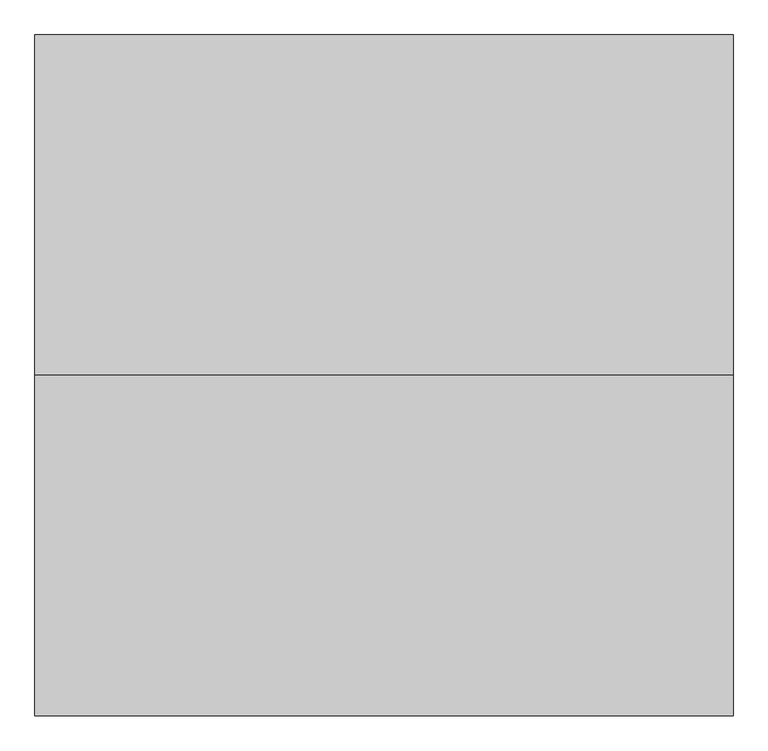
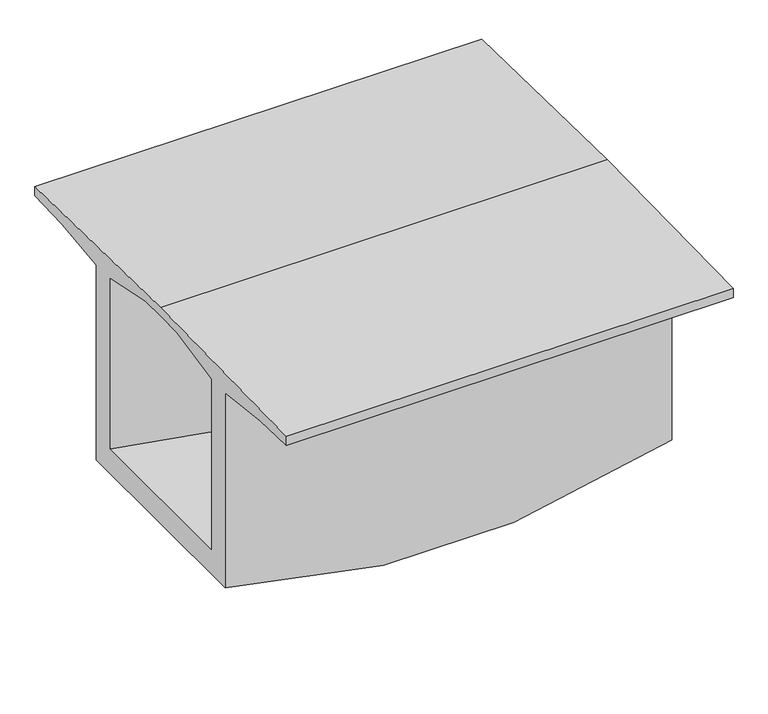
"""IFC4 building model written with IfcOpenShell, lengths in millimetres: proxy geometry, K1+K0+K1_2 : K1+K0+K1_2."""

from ifc_helpers import new_model, si_unit, frame, origin, place, context, project, spatial, source, transform, mapped, element, save
from ifc_brep_helpers import plane_surface, spline_surface, advanced_brep


def generic_models_2616fa81(model_context):
    return source(origin(), model_context, "Body", "AdvancedBrep", [
        advanced_brep(
        [(-6000.0, 5850.0, -367.0), (-6000.0, 5850.0, -117.0), (6000.0, 5850.0, -117.0), (6000.0, 5850.0, -367.0), (-6000.0, 4600.0, -421.0), (6000.0, 4599.9997971, -420.9953034), (-6000.0, 3000.0, -607.0), (6000.0, 2999.9994603, -606.9953573), (-1750.0, 3000.0, -6999.9983335), (-6000.0, 3000.0, -6150.0), (6000.0, 3000.0, -6150.0), (1750.0, 3000.0, -6999.9983335), (-1750.0, -3000.0, -6999.9983335), (-6000.0, -3000.0, -6150.0), (1750.0, -3000.0, -6999.9983335), (6000.0, -3000.0, -6150.0), (6000.0, -3000.0, -607.0), (-6000.0, -3000.0, -607.0), (-6000.0, -4600.0, -421.0), (6000.0, -4599.9994603, -420.9953573), (-6000.0, -5850.0, -367.0), (6000.0, -5849.9997971, -366.9953034), (-6000.0, -5850.0, -117.0), (6000.0, -5850.0, -117.0), (-6000.0, 0.0, 0.0), (6000.0, -9.41e-05, 0.0047035), (-6000.0, -2350.0, -5450.0), (-6000.0, 2350.0, -5450.0), (-6000.0, 2350.0, -607.0), (-6000.0, 750.0, -265.0), (-6000.0, 0.0, -250.0), (-6000.0, -750.0, -265.0), (-6000.0, -2350.0, -607.0), (-1750.0, -2100.0, -5999.9983335), (-2750.0, -2350.0, -5999.9983335), (-2750.0, -2350.0, -606.9983335), (-1750.0, -2100.0, -856.9983335), (-2750.0, -750.0, -264.9983335), (-1750.0, -750.0, -514.9983335), (-2750.0, 0.0, -249.9983335), (-1750.0, 0.0, -499.9983335), (-2750.0, 750.0, -264.9983335), (-1750.0, 750.0, -514.9983335), (-2750.0, 2350.0, -606.9983335), (-1750.0, 2100.0, -856.9983335), (-2750.0, 2350.0, -5999.9983335), (-1750.0, 2100.0, -5999.9983335), (-1750.0, 400.0, -5999.9983335), (-1750.0, 500.0, -5899.9983335), (-1750.0, 500.0, -4099.9983335), (-1750.0, 400.0, -3999.9983335), (-1750.0, -400.0, -3999.9983335), (-1750.0, -500.0, -4099.9983335), (-1750.0, -500.0, -5899.9983335), (-1750.0, -400.0, -5999.9983335), (1750.0, -400.0, -5999.9983335), (1750.0, -500.0, -5899.9983335), (1750.0, -500.0, -4099.9983335), (1750.0, -400.0, -3999.9983335), (1750.0, 400.0, -3999.9983335), (1750.0, 500.0, -4099.9983335), (1750.0, 500.0, -5899.9983335), (1750.0, 400.0, -5999.9983335), (1750.0, 2100.0, -5999.9983335), (1750.0, 2100.0, -856.9983335), (1750.0, 750.0, -514.9983335), (1750.0, 0.0, -499.9983335), (1750.0, -750.0, -514.9983335), (1750.0, -2100.0, -856.9983335), (1750.0, -2100.0, -5999.9983335), (2750.0, -2350.0, -5999.9983335), (2750.0, 2350.0, -5999.9983335), (6000.0, 2350.0, -607.0), (6000.0, 2350.0, -5450.0), (6000.0, -2350.0, -5450.0), (6000.0, -2350.0, -607.0), (6000.0, -750.0, -265.0), (6000.0, 0.0, -250.0), (6000.0, 750.0, -265.0), (2750.0, 2350.0, -606.9983335), (2750.0, 750.0, -264.9983335), (2750.0, 0.0, -249.9983335), (2750.0, -750.0, -264.9983335), (2750.0, -2350.0, -606.9983335)],
        [
            (0, 1),
            (1, 2),
            (2, 3),
            (3, 0),
            (4, 0),
            (3, 5),
            (5, 4),
            (6, 4),
            (5, 7),
            (7, 6),
            (8, 9),
            (9, 6),
            (7, 10),
            (10, 11),
            (11, 8),
            (8, 12),
            (12, 13),
            (13, 9),
            (12, 14),
            (14, 15),
            (15, 16),
            (16, 17),
            (17, 13),
            (18, 17),
            (16, 19),
            (19, 18),
            (20, 18),
            (19, 21),
            (21, 20),
            (22, 20),
            (21, 23),
            (23, 22),
            (24, 22),
            (23, 25),
            (25, 24),
            (1, 24),
            (25, 2),
            (26, 27),
            (27, 28),
            (28, 29),
            (29, 30),
            (30, 31),
            (31, 32),
            (32, 26),
            (33, 34),
            (34, 35),
            (35, 36),
            (36, 33),
            (35, 37),
            (37, 38),
            (38, 36),
            (37, 39),
            (39, 40),
            (40, 38),
            (39, 41),
            (41, 42),
            (42, 40),
            (41, 43),
            (43, 44),
            (44, 42),
            (45, 46),
            (46, 44),
            (43, 45),
            (46, 47),
            (47, 48),
            (48, 49),
            (49, 50),
            (50, 51),
            (51, 52),
            (52, 53),
            (53, 54),
            (54, 33),
            (45, 27),
            (26, 34),
            (34, 45),
            (32, 35),
            (31, 37),
            (30, 39),
            (29, 41),
            (28, 43),
            (11, 14),
            (55, 56),
            (56, 57),
            (57, 58),
            (58, 59),
            (59, 60),
            (60, 61),
            (61, 62),
            (62, 63),
            (63, 64),
            (64, 65),
            (65, 66),
            (66, 67),
            (67, 68),
            (68, 69),
            (69, 55),
            (53, 56),
            (55, 54),
            (69, 70),
            (70, 71),
            (71, 63),
            (62, 47),
            (61, 48),
            (60, 49),
            (59, 50),
            (58, 51),
            (57, 52),
            (10, 15),
            (72, 73),
            (73, 74),
            (74, 75),
            (75, 76),
            (76, 77),
            (77, 78),
            (78, 72),
            (71, 73),
            (72, 79),
            (79, 71),
            (78, 80),
            (80, 79),
            (77, 81),
            (81, 80),
            (76, 82),
            (82, 81),
            (75, 83),
            (83, 82),
            (74, 70),
            (70, 83),
            (79, 64),
            (80, 65),
            (81, 66),
            (82, 67),
            (83, 68),
        ],
        [
            plane_surface(frame((-1750.0, 5850.0, -241.9983335), z_axis=(0.0, 1.0, 0.0), x_axis=(0.0, 0.0, -1.0))),
            plane_surface(frame((-1750.0, 5225.0, -393.9983335), z_axis=(3.917521675919369e-07, 0.043159745550590725, -0.9990681840414372), x_axis=(0.0, -0.9990681840415138, -0.043159745550594035))),
            plane_surface(frame((-1750.0, 3800.0, -513.9983335), z_axis=(3.8949455357734467e-07, 0.11547236802580216, -0.9933106926950712), x_axis=(0.0, -0.9933106926951465, -0.11547236802581091))),
            plane_surface(frame((-1750.0, 3000.0, -3803.4983335), z_axis=(0.0, 1.0, 0.0), x_axis=(0.0, 0.0, -1.0))),
            plane_surface(frame((-1750.0, 0.0, -6999.9983335), z_axis=(-0.1961157654238259, 0.0, -0.9805807496337193), x_axis=(0.0, -1.0, 0.0))),
            plane_surface(frame((-1750.0, -3000.0, -3803.4983335), z_axis=(0.0, -1.0, 0.0), x_axis=(0.0, 0.0, 1.0))),
            plane_surface(frame((-1750.0, -3800.0, -513.9983335), z_axis=(3.8949455045787845e-07, -0.11547236802580199, -0.9933106926950712), x_axis=(0.0, -0.9933106926951465, 0.11547236802581075))),
            plane_surface(frame((-1750.0, -5225.0, -393.9983335), z_axis=(3.917521632228593e-07, -0.043159745550590524, -0.9990681840414372), x_axis=(0.0, -0.9990681840415138, 0.043159745550593834))),
            plane_surface(frame((-1750.0, -5850.0, -241.9983335), z_axis=(0.0, -1.0, 0.0), x_axis=(0.0, 0.0, 1.0))),
            plane_surface(frame((-1750.0, -2925.0, -58.4983335), z_axis=(-3.920391455849865e-07, -0.019996001199585858, 0.9998000599799306), x_axis=(0.0, 0.9998000599800073, 0.01999600119958739))),
            plane_surface(frame((-1750.0, 2925.0, -58.4983335), z_axis=(-3.9203914802891097e-07, 0.0199960011995859, 0.9998000599799306), x_axis=(0.0, 0.9998000599800073, -0.019996001199587433))),
            plane_surface(frame((-6000.0, 0.0, -1393.0909091), z_axis=(-1.0, 0.0, 0.0), x_axis=(0.0, 0.0, -1.0))),
            plane_surface(frame((-1750.0, -2100.0, -3428.4983335), z_axis=(-0.24253562503633255, 0.970142500145332, 0.0), x_axis=(0.0, 0.0, 1.0))),
            spline_surface(1, 1, [[(-1750.0, -2100.0, -856.9983335), (-1750.0, -750.0, -514.9983335)], [(-2750.0, -2350.0, -606.9983335), (-2750.0, -750.0, -264.9983335)]], [2, 2], [2, 2], [0.0, 1.0], [0.0, 1.0]),
            plane_surface(frame((-1750.0, -375.0, -507.4983335), z_axis=(-0.24248998415805265, 0.019399198732549593, -0.9699599366322108), x_axis=(0.0, 0.999800059980009, 0.019996001199502643))),
            plane_surface(frame((-1750.0, 375.0, -507.4983335), z_axis=(-0.2424899841580526, -0.019399198732545083, -0.969959936632211), x_axis=(0.0, 0.9998000599800091, -0.019996001199497994))),
            spline_surface(1, 1, [[(-1750.0, 750.0, -514.9983335), (-1750.0, 2100.0, -856.9983335)], [(-2750.0, 750.0, -264.9983335), (-2750.0, 2350.0, -606.9983335)]], [2, 2], [2, 2], [0.0, 1.0], [0.0, 1.0]),
            plane_surface(frame((-1750.0, 2100.0, -3428.4983335), z_axis=(-0.2425356250363329, -0.970142500145332, 0.0), x_axis=(0.0, 0.0, -1.0))),
            plane_surface(frame((-1750.0, 0.0, -2177.7126192), z_axis=(-1.0, 0.0, 0.0), x_axis=(0.0, 0.0, 1.0))),
            plane_surface(frame((-2750.0, 0.0, -5999.9983335), z_axis=(0.16685781218853318, 0.0, 0.9859809686356306), x_axis=(0.0, -1.0, 0.0))),
            plane_surface(frame((-2750.0, -2350.0, -3303.4983335), z_axis=(0.0, 1.0, 0.0), x_axis=(0.0, 0.0, 1.0))),
            plane_surface(frame((-2750.0, -1550.0, -435.9983335), z_axis=(5.014418331334979e-07, 0.2090281807047397, -0.9779096173323053), x_axis=(0.0, 0.9779096173324281, 0.20902818070476595))),
            plane_surface(frame((-2750.0, -375.0, -257.4983335), z_axis=(5.126665763907822e-07, 0.01999600119949824, -0.9998000599798776), x_axis=(0.0, 0.999800059980009, 0.019996001199500867))),
            plane_surface(frame((-2750.0, 375.0, -257.4983335), z_axis=(5.126665768021895e-07, -0.01999600119949714, -0.9998000599798776), x_axis=(0.0, 0.999800059980009, -0.019996001199499767))),
            plane_surface(frame((-2750.0, 1550.0, -435.9983335), z_axis=(5.014418348904322e-07, -0.209028180704739, -0.9779096173323053), x_axis=(0.0, 0.9779096173324282, -0.20902818070476525))),
            plane_surface(frame((-2750.0, 2350.0, -3303.4983335), z_axis=(0.0, -1.0, 0.0), x_axis=(0.0, 0.0, -1.0))),
            plane_surface(frame((-1750.0, 0.0, -6999.9983335), z_axis=(0.0, 0.0, -1.0), x_axis=(0.0, 1.0, 0.0))),
            plane_surface(frame((1750.0, 0.0, -1547.6346971), z_axis=(1.0, 0.0, 0.0), x_axis=(0.0, -0.9998000599800073, 0.019996001199585656))),
            plane_surface(frame((-1750.0, -450.0, -5949.9983335), z_axis=(0.0, 0.7071067811866191, 0.7071067811864761), x_axis=(0.0, 0.7071067811864761, -0.7071067811866191))),
            plane_surface(frame((-1750.0, 0.0, -5999.9983335), z_axis=(0.0, 0.0, 1.0), x_axis=(0.0, 1.0, 0.0))),
            plane_surface(frame((-1750.0, 450.0, -5949.9983335), z_axis=(0.0, -0.7071067811866215, 0.7071067811864736), x_axis=(0.0, 0.7071067811864736, 0.7071067811866215))),
            plane_surface(frame((-1750.0, 500.0, -4999.9983335), z_axis=(0.0, -1.0, 0.0), x_axis=(0.0, 0.0, 1.0))),
            plane_surface(frame((-1750.0, 450.0, -4049.9983335), z_axis=(0.0, -0.707106781186443, -0.7071067811866522), x_axis=(0.0, -0.7071067811866522, 0.707106781186443))),
            plane_surface(frame((-1750.0, 0.0, -3999.9983335), z_axis=(0.0, 0.0, -1.0), x_axis=(0.0, -1.0, 0.0))),
            plane_surface(frame((-1750.0, -450.0, -4049.9983335), z_axis=(0.0, 0.7071067811864454, -0.7071067811866497), x_axis=(0.0, -0.7071067811866497, -0.7071067811864454))),
            plane_surface(frame((-1750.0, -500.0, -4999.9983335), z_axis=(0.0, 1.0, 0.0), x_axis=(0.0, 0.0, -1.0))),
            plane_surface(frame((1750.0, 0.0, -6999.9983335), z_axis=(0.1961157654238259, 0.0, -0.9805807496337193), x_axis=(0.0, 1.0, 0.0))),
            plane_surface(frame((6000.0, 0.0, -1393.0909091), z_axis=(1.0000000000000002, 0.0, 0.0), x_axis=(0.0, -0.9998000599800073, 0.019996001199587433))),
            plane_surface(frame((2750.0, 2350.0, -3303.4983335), z_axis=(0.0, -1.0, 0.0), x_axis=(0.0, 0.0, 1.0))),
            plane_surface(frame((2750.0, 1550.0, -435.9983335), z_axis=(-5.014418348904322e-07, -0.209028180704739, -0.9779096173323053), x_axis=(0.0, -0.9779096173324282, 0.20902818070476525))),
            plane_surface(frame((2750.0, 375.0, -257.4983335), z_axis=(-5.126665768021895e-07, -0.01999600119949714, -0.9998000599798776), x_axis=(0.0, -0.999800059980009, 0.019996001199499767))),
            plane_surface(frame((2750.0, -375.0, -257.4983335), z_axis=(-5.126665763907822e-07, 0.01999600119949824, -0.9998000599798776), x_axis=(0.0, -0.999800059980009, -0.019996001199500867))),
            plane_surface(frame((2750.0, -1550.0, -435.9983335), z_axis=(-5.014418331334979e-07, 0.2090281807047397, -0.9779096173323053), x_axis=(0.0, -0.9779096173324281, -0.20902818070476595))),
            plane_surface(frame((2750.0, -2350.0, -3303.4983335), z_axis=(0.0, 1.0, 0.0), x_axis=(0.0, 0.0, -1.0))),
            plane_surface(frame((2750.0, 0.0, -5999.9983335), z_axis=(-0.16685781218853318, 0.0, 0.9859809686356306), x_axis=(0.0, 1.0, 0.0))),
            plane_surface(frame((1750.0, 2100.0, -3428.4983335), z_axis=(0.2425356250363329, -0.970142500145332, 0.0), x_axis=(0.0, 0.0, 1.0))),
            spline_surface(1, 1, [[(1750.0, 2100.0, -856.9983335), (1750.0, 750.0, -514.9983335)], [(2750.0, 2350.0, -606.9983335), (2750.0, 750.0, -264.9983335)]], [2, 2], [2, 2], [0.0, 1.0], [0.0, 1.0]),
            plane_surface(frame((1750.0, 375.0, -507.4983335), z_axis=(0.2424899841580526, -0.019399198732545083, -0.969959936632211), x_axis=(0.0, -0.9998000599800091, 0.019996001199497994))),
            plane_surface(frame((1750.0, -375.0, -507.4983335), z_axis=(0.24248998415805265, 0.019399198732549593, -0.9699599366322108), x_axis=(0.0, -0.999800059980009, -0.019996001199502643))),
            spline_surface(1, 1, [[(1750.0, -750.0, -514.9983335), (1750.0, -2100.0, -856.9983335)], [(2750.0, -750.0, -264.9983335), (2750.0, -2350.0, -606.9983335)]], [2, 2], [2, 2], [0.0, 1.0], [0.0, 1.0]),
            plane_surface(frame((1750.0, -2100.0, -3428.4983335), z_axis=(0.24253562503633255, 0.970142500145332, 0.0), x_axis=(0.0, 0.0, -1.0))),
        ],
        [
            (0, [[1, 2, 3, 4]]),
            (1, [[5, -4, 6, 7]]),
            (2, [[8, -7, 9, 10]]),
            (3, [[11, 12, -10, 13, 14, 15]]),
            (4, [[-11, 16, 17, 18]]),
            (5, [[-17, 19, 20, 21, 22, 23]]),
            (6, [[24, -22, 25, 26]]),
            (7, [[27, -26, 28, 29]]),
            (8, [[30, -29, 31, 32]]),
            (9, [[33, -32, 34, 35]]),
            (10, [[-2, 36, -35, 37]]),
            (11, [[-1, -5, -8, -12, -18, -23, -24, -27, -30, -33, -36], [38, 39, 40, 41, 42, 43, 44]]),
            (12, [[45, 46, 47, 48]]),
            (13, [[-47, 49, 50, 51]]),
            (14, [[-50, 52, 53, 54]]),
            (15, [[-53, 55, 56, 57]]),
            (16, [[-56, 58, 59, 60]]),
            (17, [[61, 62, -59, 63]]),
            (18, [[-48, -51, -54, -57, -60, -62, 64, 65, 66, 67, 68, 69, 70, 71, 72]]),
            (19, [[73, -38, 74, 75]]),
            (20, [[-74, -44, 76, -46]]),
            (21, [[-76, -43, 77, -49]]),
            (22, [[-77, -42, 78, -52]]),
            (23, [[-78, -41, 79, -55]]),
            (24, [[-79, -40, 80, -58]]),
            (25, [[-73, -63, -80, -39]]),
            (26, [[-19, -16, -15, 81]]),
            (27, [[82, 83, 84, 85, 86, 87, 88, 89, 90, 91, 92, 93, 94, 95, 96]]),
            (28, [[97, -82, 98, -71]]),
            (29, [[-98, -96, 99, 100, 101, -89, 102, -64, -61, -75, -45, -72]]),
            (30, [[-102, -88, 103, -65]]),
            (31, [[-103, -87, 104, -66]]),
            (32, [[-104, -86, 105, -67]]),
            (33, [[-105, -85, 106, -68]]),
            (34, [[-106, -84, 107, -69]]),
            (35, [[-97, -70, -107, -83]]),
            (36, [[-20, -81, -14, 108]]),
            (37, [[-37, -34, -31, -28, -25, -21, -108, -13, -9, -6, -3], [109, 110, 111, 112, 113, 114, 115]]),
            (38, [[116, -109, 117, 118]]),
            (39, [[-117, -115, 119, 120]]),
            (40, [[-119, -114, 121, 122]]),
            (41, [[-121, -113, 123, 124]]),
            (42, [[-123, -112, 125, 126]]),
            (43, [[-125, -111, 127, 128]]),
            (44, [[-116, -100, -127, -110]]),
            (45, [[-101, -118, 129, -90]]),
            (46, [[-129, -120, 130, -91]]),
            (47, [[-130, -122, 131, -92]]),
            (48, [[-131, -124, 132, -93]]),
            (49, [[-132, -126, 133, -94]]),
            (50, [[-133, -128, -99, -95]]),
        ],
    ),
    ])


if __name__ == "__main__":
    model = new_model("IFC4")
    model_context = context("Model", 3, world=origin())
    ifc_project = project(units=[si_unit("LENGTHUNIT", "METRE", prefix="MILLI")], contexts=[model_context])
    site = spatial("IfcSite", under=ifc_project)
    building = spatial("IfcBuilding", under=site)
    placement = place(None, origin())
    generic_models_shape = generic_models_2616fa81(model_context)
    element("IfcBuildingElementProxy", 1, Name="K1+K0+K1_2 : K1+K0+K1_2", ObjectType="K1+K0+K1_2 : K1+K0+K1_2", at=placement, inside=building, context=model_context, shape_type="MappedRepresentation", body=[
        mapped(generic_models_shape, transform((0.0, 0.0, 0.0), x_axis=(1.0, 0.0, 0.0), y_axis=(0.0, 1.0, 0.0), z_axis=(0.0, 0.0, 1.0))),
    ])
    save(model, "model.ifc")

# Revit data of these elements
# Project information
#   Project Issue Date = "Issue Date"
#   Project Status = "Project Status"
#   Client Name = "Owner"
#   Project Address = "Enter address here"
#   Project Name = "Project Name"
#   Project Number = "Project Number"
# Type "K1+K0+K1_2 : K1+K0+K1_2"
#   Vat cua dam = 100 mm
#   Kho cau = 11700 mm
#   H_MC K1 = 6150 mm
#   Doc trai BMC = 2.00%
#   Doc phai BMC = 2.00%
#   Khoang cach xien vach dam = 0 mm
#   Chieu rong vat 2 = 186 mm
#   Chieu rong vat 1 = 54 mm
#   Chieu rong phan vat dau K0 = 250 mm
#   Chieu rong cua = 1000 mm
#   Chieu day vach dam_MC K1 = 650 mm
#   Chieu day vach dam_MC K0 = 900 mm
#   Chieu day dinh ban nap_MC K1 = 250 mm
#   Chieu day day dam_MC K1 = 700 mm
#   Chieu day day dam_MC K0 = 1000 mm
#   Chieu day BMC = 250 mm
#   Chieu dai vat 3_MC K1 = 1600 mm
#   Chieu dai vat 3_MC K0 = 1350 mm
#   Chieu dai vat 2 = 1600 mm
#   Chieu dai vat 1 = 1250 mm
#   Chieu dai doan chuyen tiep = 1000 mm
#   Chieu dai dot K1 = 3250 mm
#   H_MC K0 = 7000 mm
#   Chieu cao cua = 2000 mm
#   A5 = 770.588 mm
#   A4 = 6770.588 mm
#   A3 = 229.412 mm
#   A2 = 300 mm
#   A1 = 4250 mm
#   Default Elevation = 0
